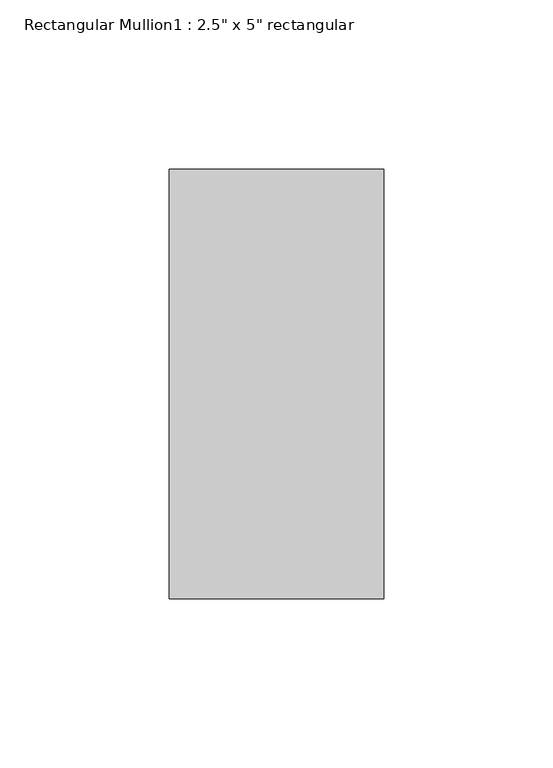
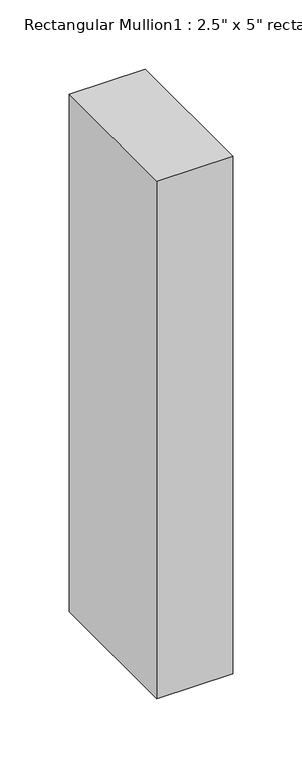
"""IFC4 building model written with IfcOpenShell, lengths in millimetres: member geometry."""

from ifc_helpers import new_model, si_unit, frame, origin, place, context, project, spatial, polyline, outline, extrude, source, transform, mapped, element, save


def member_15823cb3(model_context):
    return source(origin(), model_context, "Body", "SweptSolid", [
        extrude(outline(polyline([(0.0, 63.5), (0.0, -63.5), (-63.5, -63.5), (-63.5, 63.5), (0.0, 63.5)])), frame((0.0, 0.0, -457.2), z_axis=(0.0, 0.0, 1.0), x_axis=(1.0, 0.0, 0.0)), (0.0, 0.0, 1.0), 457.2),
    ])


if __name__ == "__main__":
    model = new_model("IFC4")
    model_context = context("Model", 3, world=origin())
    ifc_project = project(units=[si_unit("LENGTHUNIT", "METRE", prefix="MILLI")], contexts=[model_context])
    site = spatial("IfcSite", under=ifc_project)
    building = spatial("IfcBuilding", under=site)
    placement = place(None, origin())
    member_shape = member_15823cb3(model_context)
    element("IfcMember", 1, ObjectType="Rectangular Mullion1 : 2.5\" x 5\" rectangular", at=placement, inside=building, context=model_context, shape_type="MappedRepresentation", body=[
        mapped(member_shape, transform((0.0, 0.0, 0.0), x_axis=(1.0, 0.0, 0.0), y_axis=(0.0, 1.0, 0.0), z_axis=(0.0, 0.0, 1.0))),
    ])
    save(model, "model.ifc")

# Revit data of these elements
# Type "Rectangular Mullion1 : 2.5\" x 5\" rectangular"
#   built-in parameter 1007304 = 0.416667 (stored number, unit not read)
#   built-in parameter 1007301 = 0.104167 (stored number, unit not read)
#   built-in parameter 1007300 = 0.104167 (stored number, unit not read)
# Element 1 (IfcMember, "Rectangular Mullion1 : 2.5\" x 5\" rectangular")
#   Materials on its faces: "support-frame"
# Materials
#   "support-frame": class "Unassigned", colour RGB 233 233 233, transparency 0, Cost = 0
